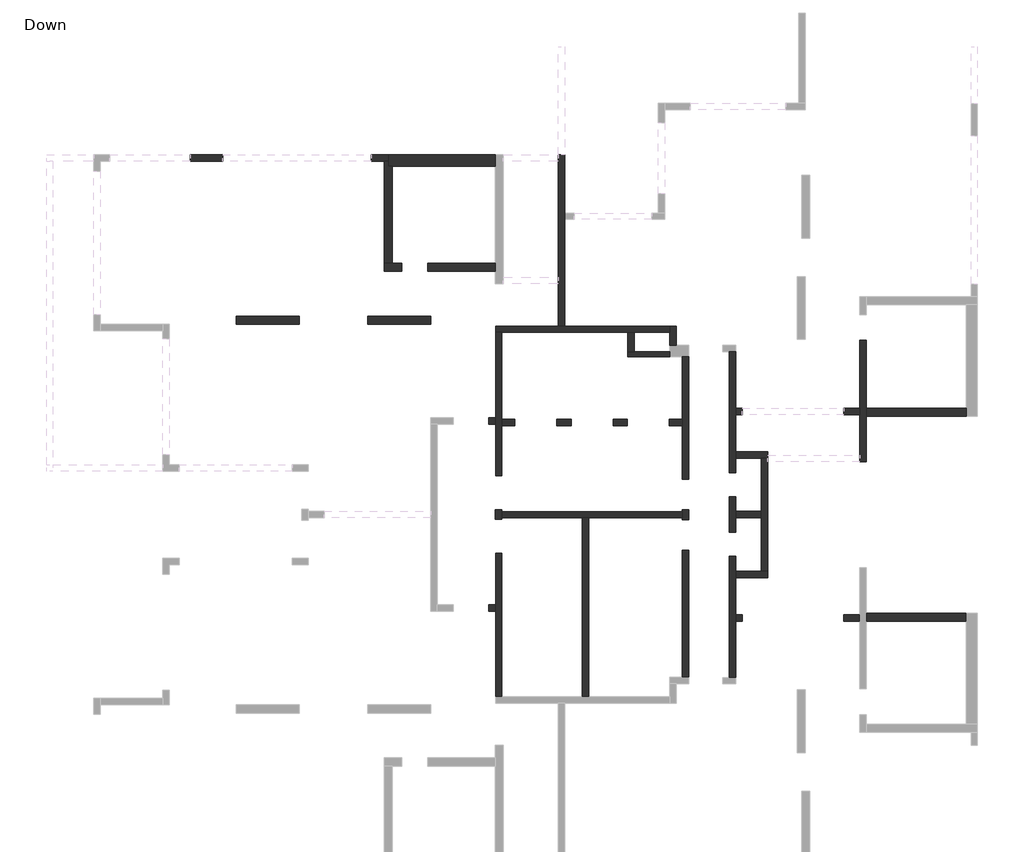
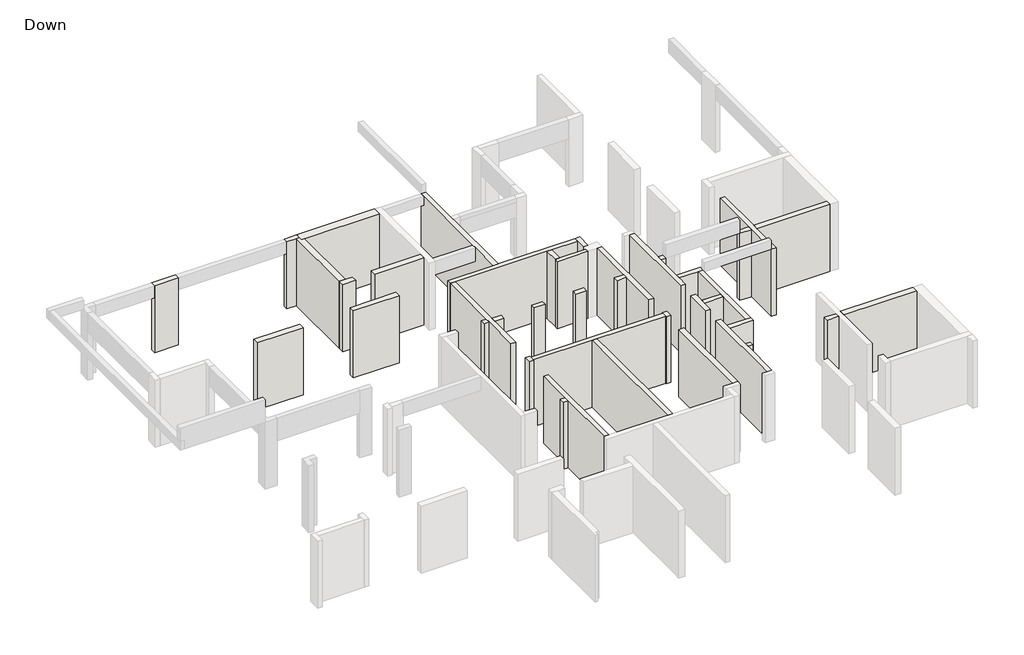
# One storey, part 2 of 3: 42 walls.
"""IFC4 building model written with IfcOpenShell, lengths in millimetres."""

from ifc_helpers import new_model, si_unit, origin, origin_with_axes, place, context, project, spatial, polyline, outline, extrude, faceted_brep, element, save

model = new_model("IFC4")

# Units and contexts
model_context = context("Model", 3, world=origin())
ifc_project = project(units=[si_unit("LENGTHUNIT", "METRE", prefix="MILLI")], contexts=[model_context])

# Site, building, storey
site = spatial("IfcSite", under=ifc_project)
building = spatial("IfcBuilding", under=site)
storey = spatial("IfcBuildingStorey", under=building, Name="Down", Elevation=0.0)

# Walls
placement = place(None, origin())
element("IfcWall", 1, ObjectType="15", at=placement, inside=storey, context=model_context, shape_type="Brep", body=[
    faceted_brep([(5701.4257984, 8540.0714033, 0.0), (4601.4257984, 8540.0714033, 0.0), (4401.4257984, 8540.0714033, 0.0), (4401.4257984, 8540.0714033, 3000.0), (4601.4257984, 8540.0714033, 3000.0), (5701.4257984, 8540.0714033, 3000.0), (5701.4257984, 8390.0714033, 0.0), (5701.4257984, 8390.0714033, 3000.0), (4401.4257984, 8390.0714033, 3000.0), (4401.4257984, 8390.0714033, 0.0)], [[[0, 1, 2, 3, 4, 5]], [[6, 7, 8, 9]], [[2, 1, 0, 6, 9]], [[5, 4, 3, 8, 7]], [[3, 2, 9, 8]], [[0, 5, 7, 6]]]),
])
element("IfcWall", 2, ObjectType="20", at=placement, inside=storey, context=model_context, shape_type="Brep", body=[
    faceted_brep([(-3022.0483227, 14641.4166181, 0.0), (-3547.0483227, 14641.4166181, 0.0), (-3547.0483227, 14641.4166181, 2450.0), (-3547.0483227, 14641.4166181, 3000.0), (-3022.0483227, 14641.4166181, 3000.0), (-3022.0483227, 14441.4166181, 0.0), (-3022.0483227, 14441.4166181, 3000.0), (-3147.0483227, 14441.4166181, 3000.0), (-3547.0483227, 14441.4166181, 3000.0), (-3547.0483227, 14441.4166181, 2450.0), (-3547.0483227, 14441.4166181, 0.0), (-3147.0483227, 14441.4166181, 0.0)], [[[0, 1, 2, 3, 4]], [[5, 6, 7, 8, 9, 10, 11]], [[1, 0, 5, 11, 10]], [[3, 2, 1, 10, 9, 8]], [[4, 3, 8, 7, 6]], [[0, 4, 6, 5]]]),
])
element("IfcWall", 3, ObjectType="20", at=placement, inside=storey, context=model_context, shape_type="Brep", body=[
    faceted_brep([(-9154.7387524, 14441.4166181, 0.0), (-8149.7387524, 14441.4166181, 0.0), (-8149.7387524, 14441.4166181, 2450.0), (-8149.7387524, 14441.4166181, 3000.0), (-9154.7387524, 14441.4166181, 3000.0), (-9154.7387524, 14441.4166181, 2450.0), (-9154.7387524, 14641.4166181, 0.0), (-9154.7387524, 14641.4166181, 2450.0), (-9154.7387524, 14641.4166181, 3000.0), (-8149.7387524, 14641.4166181, 3000.0), (-8149.7387524, 14641.4166181, 2450.0), (-8149.7387524, 14641.4166181, 0.0)], [[[0, 1, 2, 3, 4, 5]], [[6, 7, 8, 9, 10, 11]], [[1, 0, 6, 11]], [[3, 2, 1, 11, 10, 9]], [[4, 3, 9, 8]], [[0, 5, 4, 8, 7, 6]]]),
])
element("IfcWall", 4, ObjectType="20", at=placement, inside=storey, context=model_context, shape_type="Brep", body=[
    faceted_brep([(2246.4257984, 14641.4166181, 0.0), (2246.4257984, 9337.0757978, 0.0), (2246.4257984, 9337.0757978, 2820.0), (2246.4257984, 9337.0757978, 3000.0), (2246.4257984, 10641.3507002, 3000.0), (2246.4257984, 10841.3507002, 3000.0), (2246.4257984, 14441.4166181, 3000.0), (2246.4257984, 14641.4166181, 3000.0), (2246.4257984, 14641.4166181, 2750.0), (2446.4257984, 14641.4166181, 0.0), (2446.4257984, 14641.4166181, 2750.0), (2446.4257984, 14641.4166181, 3000.0), (2446.4257984, 12840.2984541, 3000.0), (2446.4257984, 12640.2984541, 3000.0), (2446.4257984, 9337.0757978, 3000.0), (2446.4257984, 9337.0757978, 2820.0), (2446.4257984, 9337.0757978, 0.0), (2446.4257984, 12640.2984541, 0.0), (2446.4257984, 12840.2984541, 0.0)], [[[0, 1, 2, 3, 4, 5, 6, 7, 8]], [[9, 10, 11, 12, 13, 14, 15, 16, 17, 18]], [[1, 0, 9, 18, 17, 16]], [[7, 6, 5, 4, 3, 14, 13, 12, 11]], [[0, 8, 7, 11, 10, 9]], [[3, 2, 1, 16, 15, 14]]]),
])
element("IfcWall", 5, ObjectType="20", at=placement, inside=storey, context=model_context, shape_type="Brep", body=[
    faceted_brep([(11596.5527515, 8889.8297041, 0.0), (11596.5527515, 6791.3653486, 0.0), (11596.5527515, 6591.3653486, 0.0), (11596.5527515, 5134.8297041, 0.0), (11596.5527515, 5134.8297041, 2820.0), (11596.5527515, 5134.8297041, 3000.0), (11596.5527515, 6591.3653486, 3000.0), (11596.5527515, 6791.3653486, 3000.0), (11596.5527515, 8889.8297041, 3000.0), (11596.5527515, 8889.8297041, 2820.0), (11796.5527515, 8889.8297041, 0.0), (11796.5527515, 8889.8297041, 2820.0), (11796.5527515, 8889.8297041, 3000.0), (11796.5527515, 6791.445915, 3000.0), (11796.5527515, 6541.445915, 3000.0), (11796.5527515, 5134.8297041, 3000.0), (11796.5527515, 5134.8297041, 0.0), (11796.5527515, 6541.445915, 0.0), (11796.5527515, 6791.445915, 0.0)], [[[0, 1, 2, 3, 4, 5, 6, 7, 8, 9]], [[10, 11, 12, 13, 14, 15, 16, 17, 18]], [[3, 2, 1, 0, 10, 18, 17, 16]], [[5, 4, 3, 16, 15]], [[8, 7, 6, 5, 15, 14, 13, 12]], [[0, 9, 8, 12, 11, 10]]]),
])
element("IfcWall", 6, ObjectType="20", at=placement, inside=storey, context=model_context, shape_type="Brep", body=[
    faceted_brep([(11103.869646, 6591.3653486, 0.0), (11596.5527515, 6591.3653486, 0.0), (11596.5527515, 6591.3653486, 2820.0), (11596.5527515, 6591.3653486, 3000.0), (11103.869646, 6591.3653486, 3000.0), (11103.869646, 6591.3653486, 2820.0), (11103.869646, 6791.3653486, 0.0), (11103.869646, 6791.3653486, 2820.0), (11103.869646, 6791.3653486, 3000.0), (11596.5527515, 6791.3653486, 3000.0), (11596.5527515, 6791.3653486, 2820.0), (11596.5527515, 6791.3653486, 0.0)], [[[0, 1, 2, 3, 4, 5]], [[6, 7, 8, 9, 10, 11]], [[1, 0, 6, 11]], [[4, 3, 9, 8]], [[0, 5, 4, 8, 7, 6]], [[3, 2, 1, 11, 10, 9]]]),
])
element("IfcWall", 7, ObjectType="20", at=placement, inside=storey, context=model_context, shape_type="Brep", body=[
    faceted_brep([(5701.4257984, 9337.0757978, 0.0), (5701.4257984, 9137.0757978, 0.0), (5701.4257984, 8740.0714033, 0.0), (5701.4257984, 8740.0714033, 3000.0), (5701.4257984, 9137.0757978, 3000.0), (5701.4257984, 9337.0757978, 3000.0), (5901.4257984, 9337.0757978, 0.0), (5901.4257984, 9337.0757978, 2820.0), (5901.4257984, 9337.0757978, 3000.0), (5901.4257984, 8740.0714033, 3000.0), (5901.4257984, 8740.0714033, 2820.0), (5901.4257984, 8740.0714033, 0.0)], [[[0, 1, 2, 3, 4, 5]], [[6, 7, 8, 9, 10, 11]], [[2, 1, 0, 6, 11]], [[5, 4, 3, 9, 8]], [[3, 2, 11, 10, 9]], [[0, 5, 8, 7, 6]]]),
])
element("IfcWall", 8, ObjectType="20", at=placement, inside=storey, context=model_context, shape_type="SweptSolid", body=[
    extrude(outline(polyline([(4601.4257984, 9137.0757978), (4601.4257984, 8540.0714033), (4401.4257984, 8540.0714033), (4401.4257984, 9137.0757978), (4601.4257984, 9137.0757978)])), origin_with_axes(), (0.0, 0.0, 1.0), 3000.0),
])
element("IfcWall", 9, ObjectType="20", at=placement, inside=storey, context=model_context, shape_type="Brep", body=[
    faceted_brep([(5701.4257984, 9337.0757978, 0.0), (2446.4257984, 9337.0757978, 0.0), (2246.4257984, 9337.0757978, 0.0), (306.4257984, 9337.0757978, 0.0), (306.4257984, 9337.0757978, 2820.0), (306.4257984, 9337.0757978, 3000.0), (2246.4257984, 9337.0757978, 3000.0), (2446.4257984, 9337.0757978, 3000.0), (5701.4257984, 9337.0757978, 3000.0), (5701.4257984, 9137.0757978, 0.0), (5701.4257984, 9137.0757978, 3000.0), (4601.4257984, 9137.0757978, 3000.0), (4401.4257984, 9137.0757978, 3000.0), (506.4257984, 9137.0757978, 3000.0), (306.4257984, 9137.0757978, 3000.0), (306.4257984, 9137.0757978, 0.0), (506.4257984, 9137.0757978, 0.0), (4401.4257984, 9137.0757978, 0.0), (4601.4257984, 9137.0757978, 0.0)], [[[0, 1, 2, 3, 4, 5, 6, 7, 8]], [[9, 10, 11, 12, 13, 14, 15, 16, 17, 18]], [[3, 2, 1, 0, 9, 18, 17, 16, 15]], [[8, 7, 6, 5, 14, 13, 12, 11, 10]], [[5, 4, 3, 15, 14]], [[0, 8, 10, 9]]]),
])
element("IfcWall", 10, ObjectType="20", at=placement, inside=storey, context=model_context, shape_type="Brep", body=[
    faceted_brep([(306.4257984, 9137.0757978, 0.0), (306.4257984, 6491.5264814, 0.0), (306.4257984, 6291.5264814, 0.0), (306.4257984, 4687.0757978, 0.0), (306.4257984, 4687.0757978, 2820.0), (306.4257984, 4687.0757978, 3000.0), (306.4257984, 6291.5264814, 3000.0), (306.4257984, 6491.5264814, 3000.0), (306.4257984, 9137.0757978, 3000.0), (506.4257984, 9137.0757978, 0.0), (506.4257984, 9137.0757978, 3000.0), (506.4257984, 6439.7589033, 3000.0), (506.4257984, 6239.7589033, 3000.0), (506.4257984, 4687.0757978, 3000.0), (506.4257984, 4687.0757978, 2820.0), (506.4257984, 4687.0757978, 0.0), (506.4257984, 6239.7589033, 0.0), (506.4257984, 6439.7589033, 0.0)], [[[0, 1, 2, 3, 4, 5, 6, 7, 8]], [[9, 10, 11, 12, 13, 14, 15, 16, 17]], [[3, 2, 1, 0, 9, 17, 16, 15]], [[5, 4, 3, 15, 14, 13]], [[8, 7, 6, 5, 13, 12, 11, 10]], [[0, 8, 10, 9]]]),
])
element("IfcWall", 11, ObjectType="20", at=placement, inside=storey, context=model_context, shape_type="Brep", body=[
    faceted_brep([(506.4257984, 6239.7589033, 0.0), (900.756853, 6239.7589033, 0.0), (900.756853, 6239.7589033, 2820.0), (900.756853, 6239.7589033, 3000.0), (506.4257984, 6239.7589033, 3000.0), (506.4257984, 6239.7589033, 2820.0), (506.4257984, 6439.7589033, 0.0), (506.4257984, 6439.7589033, 3000.0), (900.756853, 6439.7589033, 3000.0), (900.756853, 6439.7589033, 2820.0), (900.756853, 6439.7589033, 0.0)], [[[0, 1, 2, 3, 4, 5]], [[6, 7, 8, 9, 10]], [[1, 0, 6, 10]], [[3, 2, 1, 10, 9, 8]], [[4, 3, 8, 7]], [[0, 5, 4, 7, 6]]]),
])
element("IfcWall", 12, ObjectType="20", at=placement, inside=storey, context=model_context, shape_type="Brep", body=[
    faceted_brep([(306.4257984, 6491.5264814, 0.0), (96.4257984, 6491.5264814, 0.0), (96.4257984, 6491.5264814, 2820.0), (96.4257984, 6491.5264814, 3000.0), (306.4257984, 6491.5264814, 3000.0), (306.4257984, 6491.5264814, 2820.0), (306.4257984, 6291.5264814, 0.0), (306.4257984, 6291.5264814, 2820.0), (306.4257984, 6291.5264814, 3000.0), (96.4257984, 6291.5264814, 3000.0), (96.4257984, 6291.5264814, 2820.0), (96.4257984, 6291.5264814, 0.0)], [[[0, 1, 2, 3, 4, 5]], [[6, 7, 8, 9, 10, 11]], [[1, 0, 6, 11]], [[3, 2, 1, 11, 10, 9]], [[4, 3, 9, 8]], [[0, 5, 4, 8, 7, 6]]]),
])
element("IfcWall", 13, ObjectType="20", at=placement, inside=storey, context=model_context, shape_type="Brep", body=[
    faceted_brep([(2196.5063648, 6239.7589033, 0.0), (2645.7812671, 6239.7589033, 0.0), (2645.7812671, 6239.7589033, 2820.0), (2645.7812671, 6239.7589033, 3000.0), (2196.5063648, 6239.7589033, 3000.0), (2196.5063648, 6239.7589033, 2820.0), (2196.5063648, 6439.7589033, 0.0), (2196.5063648, 6439.7589033, 2820.0), (2196.5063648, 6439.7589033, 3000.0), (2645.7812671, 6439.7589033, 3000.0), (2645.7812671, 6439.7589033, 2820.0), (2645.7812671, 6439.7589033, 0.0)], [[[0, 1, 2, 3, 4, 5]], [[6, 7, 8, 9, 10, 11]], [[1, 0, 6, 11]], [[3, 2, 1, 11, 10, 9]], [[4, 3, 9, 8]], [[0, 5, 4, 8, 7, 6]]]),
])
element("IfcWall", 14, ObjectType="20", at=placement, inside=storey, context=model_context, shape_type="Brep", body=[
    faceted_brep([(3950.197771, 6239.7589033, 0.0), (4397.3022632, 6239.7589033, 0.0), (4397.3022632, 6239.7589033, 2820.0), (4397.3022632, 6239.7589033, 3000.0), (3950.197771, 6239.7589033, 3000.0), (3950.197771, 6239.7589033, 2820.0), (3950.197771, 6439.7589033, 0.0), (3950.197771, 6439.7589033, 2820.0), (3950.197771, 6439.7589033, 3000.0), (4397.3022632, 6439.7589033, 3000.0), (4397.3022632, 6439.7589033, 2820.0), (4397.3022632, 6439.7589033, 0.0)], [[[0, 1, 2, 3, 4, 5]], [[6, 7, 8, 9, 10, 11]], [[1, 0, 6, 11]], [[3, 2, 1, 11, 10, 9]], [[4, 3, 9, 8]], [[0, 5, 4, 8, 7, 6]]]),
])
element("IfcWall", 15, ObjectType="20", at=placement, inside=storey, context=model_context, shape_type="Brep", body=[
    faceted_brep([(5697.3779468, 6239.7589033, 0.0), (6096.4111499, 6239.7589033, 0.0), (6096.4111499, 6239.7589033, 2820.0), (6096.4111499, 6239.7589033, 3000.0), (5697.3779468, 6239.7589033, 3000.0), (5697.3779468, 6239.7589033, 2820.0), (5697.3779468, 6439.7589033, 0.0), (5697.3779468, 6439.7589033, 2820.0), (5697.3779468, 6439.7589033, 3000.0), (6096.4111499, 6439.7589033, 3000.0), (6096.4111499, 6439.7589033, 0.0)], [[[0, 1, 2, 3, 4, 5]], [[6, 7, 8, 9, 10]], [[1, 0, 6, 10]], [[4, 3, 9, 8]], [[0, 5, 4, 8, 7, 6]], [[3, 2, 1, 10, 9]]]),
])
element("IfcWall", 16, ObjectType="20", at=placement, inside=storey, context=model_context, shape_type="Brep", body=[
    faceted_brep([(6296.4111499, 4590.2471845, 0.0), (6296.4111499, 8390.0714033, 0.0), (6296.4111499, 8390.0714033, 3000.0), (6296.4111499, 4590.2471845, 3000.0), (6296.4111499, 4590.2471845, 2820.0), (6096.4111499, 4590.2471845, 0.0), (6096.4111499, 4590.2471845, 2820.0), (6096.4111499, 4590.2471845, 3000.0), (6096.4111499, 6239.7589033, 3000.0), (6096.4111499, 6439.7589033, 3000.0), (6096.4111499, 8390.0714033, 3000.0), (6096.4111499, 8390.0714033, 0.0), (6096.4111499, 6439.7589033, 0.0), (6096.4111499, 6239.7589033, 0.0)], [[[0, 1, 2, 3, 4]], [[5, 6, 7, 8, 9, 10, 11, 12, 13]], [[1, 0, 5, 13, 12, 11]], [[3, 2, 10, 9, 8, 7]], [[0, 4, 3, 7, 6, 5]], [[2, 1, 11, 10]]]),
])
element("IfcWall", 17, ObjectType="20", at=placement, inside=storey, context=model_context, shape_type="Brep", body=[
    faceted_brep([(7551.2304859, 8540.3936689, 0.0), (7551.2304859, 4780.3936689, 0.0), (7551.2304859, 4780.3936689, 2820.0), (7551.2304859, 4780.3936689, 3000.0), (7551.2304859, 8540.3936689, 3000.0), (7551.2304859, 8540.3936689, 2820.0), (7751.2304859, 8540.3936689, 0.0), (7751.2304859, 8540.3936689, 3000.0), (7751.2304859, 6791.3653486, 3000.0), (7751.2304859, 6591.3653486, 3000.0), (7751.2304859, 5441.3702314, 3000.0), (7751.2304859, 5241.3702314, 3000.0), (7751.2304859, 4780.3936689, 3000.0), (7751.2304859, 4780.3936689, 2820.0), (7751.2304859, 4780.3936689, 0.0), (7751.2304859, 5241.3702314, 0.0), (7751.2304859, 5441.3702314, 0.0), (7751.2304859, 6591.3653486, 0.0), (7751.2304859, 6791.3653486, 0.0)], [[[0, 1, 2, 3, 4, 5]], [[6, 7, 8, 9, 10, 11, 12, 13, 14, 15, 16, 17, 18]], [[1, 0, 6, 18, 17, 16, 15, 14]], [[3, 2, 1, 14, 13, 12]], [[4, 3, 12, 11, 10, 9, 8, 7]], [[0, 5, 4, 7, 6]]]),
])
element("IfcWall", 18, ObjectType="20", at=placement, inside=storey, context=model_context, shape_type="Brep", body=[
    faceted_brep([(7751.2304859, 5241.3702314, 0.0), (8550.5859546, 5241.3702314, 0.0), (8750.5859546, 5241.3702314, 0.0), (8750.5859546, 5241.3702314, 3000.0), (8550.5859546, 5241.3702314, 3000.0), (7751.2304859, 5241.3702314, 3000.0), (7751.2304859, 5241.3702314, 2820.0), (7751.2304859, 5441.3702314, 0.0), (7751.2304859, 5441.3702314, 2820.0), (7751.2304859, 5441.3702314, 3000.0), (8750.5859546, 5441.3702314, 3000.0), (8750.5859546, 5441.3702314, 2820.0), (8750.5859546, 5441.3702314, 0.0)], [[[0, 1, 2, 3, 4, 5, 6]], [[7, 8, 9, 10, 11, 12]], [[2, 1, 0, 7, 12]], [[5, 4, 3, 10, 9]], [[0, 6, 5, 9, 8, 7]], [[3, 2, 12, 11, 10]]]),
])
element("IfcWall", 19, ObjectType="20", at=placement, inside=storey, context=model_context, shape_type="Brep", body=[
    faceted_brep([(8550.5859546, 5241.3702314, 0.0), (8550.5859546, 3593.6505048, 0.0), (8550.5859546, 3586.3702314, 0.0), (8550.5859546, 3386.3702314, 0.0), (8550.5859546, 1738.6505048, 0.0), (8550.5859546, 1738.6505048, 2820.0), (8550.5859546, 1738.6505048, 3000.0), (8550.5859546, 3386.3702314, 3000.0), (8550.5859546, 3586.3702314, 3000.0), (8550.5859546, 3593.6505048, 3000.0), (8550.5859546, 5241.3702314, 3000.0), (8550.5859546, 5241.3702314, 2820.0), (8750.5859546, 5241.3702314, 0.0), (8750.5859546, 5241.3702314, 3000.0), (8750.5859546, 5134.8297041, 3000.0), (8750.5859546, 1845.1910322, 3000.0), (8750.5859546, 1738.6505048, 3000.0), (8750.5859546, 1738.6505048, 0.0)], [[[0, 1, 2, 3, 4, 5, 6, 7, 8, 9, 10, 11]], [[12, 13, 14, 15, 16, 17]], [[4, 3, 2, 1, 0, 12, 17]], [[10, 9, 8, 7, 6, 16, 15, 14, 13]], [[0, 11, 10, 13, 12]], [[6, 5, 4, 17, 16]]]),
])
element("IfcWall", 20, ObjectType="20", at=placement, inside=storey, context=model_context, shape_type="Brep", body=[
    faceted_brep([(8550.5859546, 3586.3702314, 0.0), (7750.5859546, 3586.3702314, 0.0), (7750.5859546, 3586.3702314, 3000.0), (8550.5859546, 3586.3702314, 3000.0), (8550.5859546, 3386.3702314, 0.0), (8550.5859546, 3386.3702314, 2820.0), (8550.5859546, 3386.3702314, 3000.0), (7750.5859546, 3386.3702314, 3000.0), (7750.5859546, 3386.3702314, 2820.0), (7750.5859546, 3386.3702314, 0.0)], [[[0, 1, 2, 3]], [[4, 5, 6, 7, 8, 9]], [[1, 0, 4, 9]], [[3, 2, 7, 6]], [[0, 3, 6, 5, 4]], [[2, 1, 9, 8, 7]]]),
])
element("IfcWall", 21, ObjectType="20", at=placement, inside=storey, context=model_context, shape_type="Brep", body=[
    faceted_brep([(7750.5859546, 2943.6505048, 0.0), (7750.5859546, 3386.3702314, 0.0), (7750.5859546, 3586.3702314, 0.0), (7750.5859546, 3593.6505048, 0.0), (7750.5859546, 4036.3702314, 0.0), (7750.5859546, 4036.3702314, 2820.0), (7750.5859546, 4036.3702314, 3000.0), (7750.5859546, 3593.6505048, 3000.0), (7750.5859546, 3586.3702314, 3000.0), (7750.5859546, 3386.3702314, 3000.0), (7750.5859546, 2943.6505048, 3000.0), (7750.5859546, 2943.6505048, 2820.0), (7550.5859546, 2943.6505048, 0.0), (7550.5859546, 2943.6505048, 2820.0), (7550.5859546, 2943.6505048, 3000.0), (7550.5859546, 4036.3702314, 3000.0), (7550.5859546, 4036.3702314, 2820.0), (7550.5859546, 4036.3702314, 0.0)], [[[0, 1, 2, 3, 4, 5, 6, 7, 8, 9, 10, 11]], [[12, 13, 14, 15, 16, 17]], [[4, 3, 2, 1, 0, 12, 17]], [[6, 5, 4, 17, 16, 15]], [[10, 9, 8, 7, 6, 15, 14]], [[0, 11, 10, 14, 13, 12]]]),
])
element("IfcWall", 22, ObjectType="20", at=placement, inside=storey, context=model_context, shape_type="Brep", body=[
    faceted_brep([(7751.2304859, 6591.3653486, 0.0), (7955.5859546, 6591.3653486, 0.0), (7955.5859546, 6591.3653486, 2820.0), (7955.5859546, 6591.3653486, 3000.0), (7751.2304859, 6591.3653486, 3000.0), (7751.2304859, 6591.3653486, 2820.0), (7751.2304859, 6791.3653486, 0.0), (7751.2304859, 6791.3653486, 2820.0), (7751.2304859, 6791.3653486, 3000.0), (7955.5859546, 6791.3653486, 3000.0), (7955.5859546, 6791.3653486, 2820.0), (7955.5859546, 6791.3653486, 0.0)], [[[0, 1, 2, 3, 4, 5]], [[6, 7, 8, 9, 10, 11]], [[1, 0, 6, 11]], [[3, 2, 1, 11, 10, 9]], [[4, 3, 9, 8]], [[0, 5, 4, 8, 7, 6]]]),
])
element("IfcWall", 23, ObjectType="20", at=placement, inside=storey, context=model_context, shape_type="Brep", body=[
    faceted_brep([(11103.869646, 188.6553877, 0.0), (11596.5527515, 188.6553877, 0.0), (11596.5527515, 188.6553877, 2820.0), (11596.5527515, 188.6553877, 3000.0), (11103.869646, 188.6553877, 3000.0), (11103.869646, 188.6553877, 2820.0), (11103.869646, 388.6553877, 0.0), (11103.869646, 388.6553877, 2820.0), (11103.869646, 388.6553877, 3000.0), (11596.5527515, 388.6553877, 3000.0), (11596.5527515, 388.6553877, 0.0)], [[[0, 1, 2, 3, 4, 5]], [[6, 7, 8, 9, 10]], [[1, 0, 6, 10]], [[4, 3, 9, 8]], [[0, 5, 4, 8, 7, 6]], [[3, 2, 1, 10, 9]]]),
])
element("IfcWall", 24, ObjectType="20", at=placement, inside=storey, context=model_context, shape_type="Brep", body=[
    faceted_brep([(506.4257984, -2157.0550616, 0.0), (506.4257984, 2292.9449384, 0.0), (506.4257984, 2292.9449384, 3000.0), (506.4257984, -2157.0550616, 3000.0), (306.4257984, -2157.0550616, 0.0), (306.4257984, -2157.0550616, 3000.0), (306.4257984, 488.4942548, 3000.0), (306.4257984, 688.4942548, 3000.0), (306.4257984, 2292.9449384, 3000.0), (306.4257984, 2292.9449384, 2820.0), (306.4257984, 2292.9449384, 0.0), (306.4257984, 688.4942548, 0.0), (306.4257984, 488.4942548, 0.0)], [[[0, 1, 2, 3]], [[4, 5, 6, 7, 8, 9, 10, 11, 12]], [[1, 0, 4, 12, 11, 10]], [[2, 1, 10, 9, 8]], [[3, 2, 8, 7, 6, 5]], [[0, 3, 5, 4]]]),
])
element("IfcWall", 25, ObjectType="20", at=placement, inside=storey, context=model_context, shape_type="Brep", body=[
    faceted_brep([(306.4257984, 688.4942548, 0.0), (96.4257984, 688.4942548, 0.0), (96.4257984, 688.4942548, 2820.0), (96.4257984, 688.4942548, 3000.0), (306.4257984, 688.4942548, 3000.0), (306.4257984, 688.4942548, 2820.0), (306.4257984, 488.4942548, 0.0), (306.4257984, 488.4942548, 2820.0), (306.4257984, 488.4942548, 3000.0), (96.4257984, 488.4942548, 3000.0), (96.4257984, 488.4942548, 2820.0), (96.4257984, 488.4942548, 0.0)], [[[0, 1, 2, 3, 4, 5]], [[6, 7, 8, 9, 10, 11]], [[1, 0, 6, 11]], [[3, 2, 1, 11, 10, 9]], [[4, 3, 9, 8]], [[0, 5, 4, 8, 7, 6]]]),
])
element("IfcWall", 26, ObjectType="20", at=placement, inside=storey, context=model_context, shape_type="Brep", body=[
    faceted_brep([(6096.4111499, 2389.7735517, 0.0), (6096.4111499, -1559.7284014, 0.0), (6096.4111499, -1559.7284014, 3000.0), (6096.4111499, 2389.4512861, 3000.0), (6096.4111499, 2389.7735517, 3000.0), (6096.4111499, 2389.7735517, 2820.0), (6296.4111499, 2389.7735517, 0.0), (6296.4111499, 2389.7735517, 2820.0), (6296.4111499, 2389.7735517, 3000.0), (6296.4111499, -1559.7284014, 3000.0), (6296.4111499, -1559.7284014, 0.0)], [[[0, 1, 2, 3, 4, 5]], [[6, 7, 8, 9, 10]], [[1, 0, 6, 10]], [[4, 3, 2, 9, 8]], [[0, 5, 4, 8, 7, 6]], [[2, 1, 10, 9]]]),
])
element("IfcWall", 27, ObjectType="20", at=placement, inside=storey, context=model_context, shape_type="Brep", body=[
    faceted_brep([(7751.2304859, -1560.3729327, 0.0), (7751.2304859, 188.6553877, 0.0), (7751.2304859, 388.6553877, 0.0), (7751.2304859, 1538.6505048, 0.0), (7751.2304859, 1738.6505048, 0.0), (7751.2304859, 2199.6270673, 0.0), (7751.2304859, 2199.6270673, 2820.0), (7751.2304859, 2199.6270673, 3000.0), (7751.2304859, 1738.6505048, 3000.0), (7751.2304859, 1538.6505048, 3000.0), (7751.2304859, 388.6553877, 3000.0), (7751.2304859, 188.6553877, 3000.0), (7751.2304859, -1560.3729327, 3000.0), (7551.2304859, -1560.3729327, 0.0), (7551.2304859, -1560.3729327, 3000.0), (7551.2304859, 2199.6270673, 3000.0), (7551.2304859, 2199.6270673, 2820.0), (7551.2304859, 2199.6270673, 0.0)], [[[0, 1, 2, 3, 4, 5, 6, 7, 8, 9, 10, 11, 12]], [[13, 14, 15, 16, 17]], [[5, 4, 3, 2, 1, 0, 13, 17]], [[7, 6, 5, 17, 16, 15]], [[12, 11, 10, 9, 8, 7, 15, 14]], [[0, 12, 14, 13]]]),
])
element("IfcWall", 28, ObjectType="20", at=placement, inside=storey, context=model_context, shape_type="Brep", body=[
    faceted_brep([(7751.2304859, 1538.6505048, 0.0), (8750.5859546, 1538.6505048, 0.0), (8750.5859546, 1538.6505048, 2820.0), (8750.5859546, 1538.6505048, 3000.0), (7751.2304859, 1538.6505048, 3000.0), (7751.2304859, 1538.6505048, 2820.0), (7751.2304859, 1738.6505048, 0.0), (7751.2304859, 1738.6505048, 2820.0), (7751.2304859, 1738.6505048, 3000.0), (8550.5859546, 1738.6505048, 3000.0), (8750.5859546, 1738.6505048, 3000.0), (8750.5859546, 1738.6505048, 0.0), (8550.5859546, 1738.6505048, 0.0)], [[[0, 1, 2, 3, 4, 5]], [[6, 7, 8, 9, 10, 11, 12]], [[1, 0, 6, 12, 11]], [[4, 3, 10, 9, 8]], [[0, 5, 4, 8, 7, 6]], [[3, 2, 1, 11, 10]]]),
])
element("IfcWall", 29, ObjectType="20", at=placement, inside=storey, context=model_context, shape_type="Brep", body=[
    faceted_brep([(8550.5859546, 3593.6505048, 0.0), (7750.5859546, 3593.6505048, 0.0), (7750.5859546, 3593.6505048, 2820.0), (7750.5859546, 3593.6505048, 3000.0), (8550.5859546, 3593.6505048, 3000.0), (8550.5859546, 3593.6505048, 2820.0), (8550.5859546, 3586.3702314, 0.0), (7750.5859546, 3586.3702314, 0.0), (7750.5859546, 3586.3702314, 3000.0), (8550.5859546, 3586.3702314, 3000.0)], [[[0, 1, 2, 3, 4, 5]], [[1, 0, 6, 7]], [[4, 3, 8, 9]], [[0, 5, 4, 9, 6]], [[3, 2, 1, 7, 8]], [[7, 6, 9, 8]]]),
])
element("IfcWall", 30, ObjectType="20", at=placement, inside=storey, context=model_context, shape_type="Brep", body=[
    faceted_brep([(7751.2304859, 188.6553877, 0.0), (7955.5859546, 188.6553877, 0.0), (7955.5859546, 188.6553877, 2820.0), (7955.5859546, 188.6553877, 3000.0), (7751.2304859, 188.6553877, 3000.0), (7751.2304859, 188.6553877, 2820.0), (7751.2304859, 388.6553877, 0.0), (7751.2304859, 388.6553877, 2820.0), (7751.2304859, 388.6553877, 3000.0), (7955.5859546, 388.6553877, 3000.0), (7955.5859546, 388.6553877, 2820.0), (7955.5859546, 388.6553877, 0.0)], [[[0, 1, 2, 3, 4, 5]], [[6, 7, 8, 9, 10, 11]], [[1, 0, 6, 11]], [[3, 2, 1, 11, 10, 9]], [[4, 3, 9, 8]], [[0, 5, 4, 8, 7, 6]]]),
])
element("IfcWall", 31, ObjectType="20", at=placement, inside=storey, context=model_context, shape_type="Brep", body=[
    faceted_brep([(501.7382984, 3340.0909345, 0.0), (501.7382984, 3385.0909345, 0.0), (501.7382984, 3585.0909345, 0.0), (501.7382984, 3635.0909345, 0.0), (501.7382984, 3635.0909345, 2820.0), (501.7382984, 3635.0909345, 3000.0), (501.7382984, 3585.0909345, 3000.0), (501.7382984, 3385.0909345, 3000.0), (501.7382984, 3340.0909345, 3000.0), (501.7382984, 3340.0909345, 2820.0), (301.7382984, 3340.0909345, 0.0), (301.7382984, 3340.0909345, 2820.0), (301.7382984, 3340.0909345, 3000.0), (301.7382984, 3635.0909345, 3000.0), (301.7382984, 3635.0909345, 2820.0), (301.7382984, 3635.0909345, 0.0), (306.4257984, 3635.0909345, 3000.0)], [[[0, 1, 2, 3, 4, 5, 6, 7, 8, 9]], [[10, 11, 12, 13, 14, 15]], [[3, 2, 1, 0, 10, 15]], [[5, 4, 3, 15, 14, 13, 16]], [[8, 7, 6, 5, 16, 13, 12]], [[0, 9, 8, 12, 11, 10]]]),
])
element("IfcWall", 32, ObjectType="20", at=placement, inside=storey, context=model_context, shape_type="Brep", body=[
    faceted_brep([(501.7382984, 3385.0909345, 0.0), (2997.0654468, 3385.0909345, 0.0), (3197.0654468, 3385.0909345, 0.0), (6101.7382984, 3385.0909345, 0.0), (6101.7382984, 3385.0909345, 2820.0), (6101.7382984, 3385.0909345, 3000.0), (3197.0654468, 3385.0909345, 3000.0), (2997.0654468, 3385.0909345, 3000.0), (501.7382984, 3385.0909345, 3000.0), (501.7382984, 3385.0909345, 2820.0), (501.7382984, 3585.0909345, 0.0), (501.7382984, 3585.0909345, 2820.0), (501.7382984, 3585.0909345, 3000.0), (6101.7382984, 3585.0909345, 3000.0), (6101.7382984, 3585.0909345, 2820.0), (6101.7382984, 3585.0909345, 0.0)], [[[0, 1, 2, 3, 4, 5, 6, 7, 8, 9]], [[10, 11, 12, 13, 14, 15]], [[3, 2, 1, 0, 10, 15]], [[8, 7, 6, 5, 13, 12]], [[0, 9, 8, 12, 11, 10]], [[5, 4, 3, 15, 14, 13]]]),
])
element("IfcWall", 33, ObjectType="20", at=placement, inside=storey, context=model_context, shape_type="Brep", body=[
    faceted_brep([(6301.7382984, 3335.0909345, 0.0), (6301.7382984, 3635.0909345, 0.0), (6301.7382984, 3635.0909345, 2820.0), (6301.7382984, 3635.0909345, 3000.0), (6301.7382984, 3335.0909345, 3000.0), (6301.7382984, 3335.0909345, 2820.0), (6101.7382984, 3335.0909345, 0.0), (6101.7382984, 3335.0909345, 2820.0), (6101.7382984, 3335.0909345, 3000.0), (6101.7382984, 3385.0909345, 3000.0), (6101.7382984, 3585.0909345, 3000.0), (6101.7382984, 3635.0909345, 3000.0), (6101.7382984, 3635.0909345, 2820.0), (6101.7382984, 3635.0909345, 0.0), (6101.7382984, 3585.0909345, 0.0), (6101.7382984, 3385.0909345, 0.0), (6296.4111499, 3635.0909345, 3000.0)], [[[0, 1, 2, 3, 4, 5]], [[6, 7, 8, 9, 10, 11, 12, 13, 14, 15]], [[1, 0, 6, 15, 14, 13]], [[3, 2, 1, 13, 12, 11, 16]], [[4, 3, 16, 11, 10, 9, 8]], [[0, 5, 4, 8, 7, 6]]]),
])
element("IfcWall", 34, ObjectType="20", at=placement, inside=storey, context=model_context, shape_type="Brep", body=[
    faceted_brep([(2997.0654468, 3385.0909345, 0.0), (2997.0654468, -2157.0550616, 0.0), (2997.0654468, -2157.0550616, 3000.0), (2997.0654468, 2292.9449384, 3000.0), (2997.0654468, 3385.0909345, 3000.0), (2997.0654468, 3385.0909345, 2820.0), (3197.0654468, 3385.0909345, 0.0), (3197.0654468, 3385.0909345, 2820.0), (3197.0654468, 3385.0909345, 3000.0), (3197.0654468, 2389.4512861, 3000.0), (3197.0654468, -2157.0550616, 3000.0), (3197.0654468, -2157.0550616, 0.0)], [[[0, 1, 2, 3, 4, 5]], [[6, 7, 8, 9, 10, 11]], [[1, 0, 6, 11]], [[4, 3, 2, 10, 9, 8]], [[0, 5, 4, 8, 7, 6]], [[2, 1, 11, 10]]]),
])
element("IfcWall", 35, ObjectType="25", at=placement, inside=storey, context=model_context, shape_type="Brep", body=[
    faceted_brep([(-7730.9496899, 9391.1944502, 0.0), (-5784.0917798, 9391.1944502, 0.0), (-5784.0917798, 9391.1944502, 2820.0), (-5784.0917798, 9391.1944502, 3000.0), (-7730.9496899, 9391.1944502, 3000.0), (-7730.9496899, 9391.1944502, 2820.0), (-7730.9496899, 9641.1944502, 0.0), (-7730.9496899, 9641.1944502, 2820.0), (-7730.9496899, 9641.1944502, 3000.0), (-5784.0917798, 9641.1944502, 3000.0), (-5784.0917798, 9641.1944502, 2820.0), (-5784.0917798, 9641.1944502, 0.0)], [[[0, 1, 2, 3, 4, 5]], [[6, 7, 8, 9, 10, 11]], [[1, 0, 6, 11]], [[3, 2, 1, 11, 10, 9]], [[4, 3, 9, 8]], [[0, 5, 4, 8, 7, 6]]]),
])
element("IfcWall", 36, ObjectType="25", at=placement, inside=storey, context=model_context, shape_type="Brep", body=[
    faceted_brep([(-3648.408186, 9391.1944502, 0.0), (-1703.720686, 9391.1944502, 0.0), (-1703.720686, 9391.1944502, 2820.0), (-1703.720686, 9391.1944502, 3000.0), (-3648.408186, 9391.1944502, 3000.0), (-3648.408186, 9391.1944502, 2820.0), (-3648.408186, 9641.1944502, 0.0), (-3648.408186, 9641.1944502, 2820.0), (-3648.408186, 9641.1944502, 3000.0), (-1703.720686, 9641.1944502, 3000.0), (-1703.720686, 9641.1944502, 2820.0), (-1703.720686, 9641.1944502, 0.0)], [[[0, 1, 2, 3, 4, 5]], [[6, 7, 8, 9, 10, 11]], [[1, 0, 6, 11]], [[3, 2, 1, 11, 10, 9]], [[4, 3, 9, 8]], [[0, 5, 4, 8, 7, 6]]]),
])
element("IfcWall", 37, ObjectType="25", at=placement, inside=storey, context=model_context, shape_type="Brep", body=[
    faceted_brep([(-1797.0483227, 11035.7061689, 0.0), (292.9516773, 11035.7061689, 0.0), (292.9516773, 11035.7061689, 2820.0), (292.9516773, 11035.7061689, 3000.0), (-1797.0483227, 11035.7061689, 3000.0), (-1797.0483227, 11035.7061689, 2820.0), (-1797.0483227, 11285.7061689, 0.0), (-1797.0483227, 11285.7061689, 2820.0), (-1797.0483227, 11285.7061689, 3000.0), (292.9516773, 11285.7061689, 3000.0), (292.9516773, 11285.7061689, 2820.0), (292.9516773, 11285.7061689, 0.0)], [[[0, 1, 2, 3, 4, 5]], [[6, 7, 8, 9, 10, 11]], [[1, 0, 6, 11]], [[4, 3, 9, 8]], [[0, 5, 4, 8, 7, 6]], [[3, 2, 1, 11, 10, 9]]]),
])
element("IfcWall", 38, ObjectType="25", at=placement, inside=storey, context=model_context, shape_type="Brep", body=[
    faceted_brep([(-3147.0483227, 14441.4166181, 0.0), (-3147.0483227, 11285.7061689, 0.0), (-3147.0483227, 11285.7061689, 3000.0), (-3147.0483227, 14441.4166181, 3000.0), (-3147.0483227, 14441.4166181, 2820.0), (-2897.0483227, 14291.4166181, 0.0), (-2897.0483227, 14291.4166181, 2820.0), (-2897.0483227, 14291.4166181, 3000.0), (-2897.0483227, 11285.7061689, 3000.0), (-2897.0483227, 11285.7061689, 2820.0), (-2897.0483227, 11285.7061689, 0.0), (-3022.0483227, 14441.4166181, 0.0), (-3022.0483227, 14291.4166181, 0.0), (-3022.0483227, 14291.4166181, 3000.0), (-3022.0483227, 14441.4166181, 3000.0)], [[[0, 1, 2, 3, 4]], [[5, 6, 7, 8, 9, 10]], [[1, 0, 11, 12, 5, 10]], [[3, 2, 8, 7, 13, 14]], [[0, 4, 3, 14, 11]], [[14, 13, 12, 11]], [[13, 7, 6, 5, 12]], [[2, 1, 10, 9, 8]]]),
])
element("IfcWall", 39, ObjectType="25", at=placement, inside=storey, context=model_context, shape_type="Brep", body=[
    faceted_brep([(-3147.0483227, 11035.7061689, 0.0), (-2602.0483227, 11035.7061689, 0.0), (-2602.0483227, 11035.7061689, 2820.0), (-2602.0483227, 11035.7061689, 3000.0), (-3147.0483227, 11035.7061689, 3000.0), (-3147.0483227, 11035.7061689, 2820.0), (-3147.0483227, 11285.7061689, 0.0), (-3147.0483227, 11285.7061689, 3000.0), (-2897.0483227, 11285.7061689, 3000.0), (-2602.0483227, 11285.7061689, 3000.0), (-2602.0483227, 11285.7061689, 2820.0), (-2602.0483227, 11285.7061689, 0.0), (-2897.0483227, 11285.7061689, 0.0)], [[[0, 1, 2, 3, 4, 5]], [[6, 7, 8, 9, 10, 11, 12]], [[1, 0, 6, 12, 11]], [[3, 2, 1, 11, 10, 9]], [[4, 3, 9, 8, 7]], [[0, 5, 4, 7, 6]]]),
])
element("IfcWall", 40, ObjectType="25", at=placement, inside=storey, context=model_context, shape_type="Brep", body=[
    faceted_brep([(14897.1826343, 6791.445915, 0.0), (11796.5527515, 6791.445915, 0.0), (11796.5527515, 6791.445915, 2820.0), (11796.5527515, 6791.445915, 3000.0), (14897.1826343, 6791.445915, 3000.0), (14897.1826343, 6791.445915, 2820.0), (14897.1826343, 6541.445915, 0.0), (14897.1826343, 6541.445915, 3000.0), (11796.5527515, 6541.445915, 3000.0), (11796.5527515, 6541.445915, 0.0)], [[[0, 1, 2, 3, 4, 5]], [[6, 7, 8, 9]], [[1, 0, 6, 9]], [[4, 3, 8, 7]], [[0, 5, 4, 7, 6]], [[3, 2, 1, 9, 8]]]),
])
element("IfcWall", 41, ObjectType="25", at=placement, inside=storey, context=model_context, shape_type="Brep", body=[
    faceted_brep([(14897.1826343, 438.5748212, 0.0), (11796.5527515, 438.5748212, 0.0), (11796.5527515, 438.5748212, 3000.0), (14897.1826343, 438.5748212, 3000.0), (14897.1826343, 188.5748212, 0.0), (14897.1826343, 188.5748212, 2820.0), (14897.1826343, 188.5748212, 3000.0), (11796.5527515, 188.5748212, 3000.0), (11796.5527515, 188.5748212, 2820.0), (11796.5527515, 188.5748212, 0.0)], [[[0, 1, 2, 3]], [[4, 5, 6, 7, 8, 9]], [[1, 0, 4, 9]], [[3, 2, 7, 6]], [[0, 3, 6, 5, 4]], [[2, 1, 9, 8, 7]]]),
])
element("IfcWall", 42, ObjectType="35", at=placement, inside=storey, context=model_context, shape_type="Brep", body=[
    faceted_brep([(292.9516773, 14641.4166181, 0.0), (-3022.0483227, 14641.4166181, 0.0), (-3022.0483227, 14641.4166181, 3000.0), (292.9516773, 14641.4166181, 3000.0), (292.9516773, 14291.4166181, 0.0), (292.9516773, 14291.4166181, 2820.0), (292.9516773, 14291.4166181, 3000.0), (-2897.0483227, 14291.4166181, 3000.0), (-3022.0483227, 14291.4166181, 3000.0), (-3022.0483227, 14291.4166181, 0.0), (-2897.0483227, 14291.4166181, 0.0), (-3022.0483227, 14441.4166181, 0.0), (-3022.0483227, 14441.4166181, 3000.0)], [[[0, 1, 2, 3]], [[4, 5, 6, 7, 8, 9, 10]], [[1, 0, 4, 10, 9, 11]], [[2, 1, 11, 9, 8, 12]], [[3, 2, 12, 8, 7, 6]], [[0, 3, 6, 5, 4]]]),
])

save(model, "model.ifc")

# Revit data of these elements
# Type "15"
#   Layers, outside or top first: 15 cm "Concrete" (function 1)
# Type "20"
#   Layers, outside or top first: 20 cm "Concrete" (function 1)
# Type "25"
#   Layers, outside or top first: 25 cm "Concrete" (function 1)
# Type "35"
#   Layers, outside or top first: 35 cm "Concrete" (function 1)
# Element 1 (IfcWall, "15")
#   Comments = ""
#   Mark = "W112"
#   SOFiSTiK_EdgeZones = "W112"
#   SOFiSTiK_AMG_Comments = ""
#   Top Offset = 0 cm
#   Base Offset = 0 cm
#   wall height = 300 cm
#   SOFiSTiK_AMG_Scheduled = yes
#   SOFiSTiK_AMG_Adjusted = yes
#   Phase Created = New Construction
#   Base Constraint = Down
#   Top Constraint = Typical Floor
#   Materials on its faces: "Concrete"
# Element 2 (IfcWall, "20")
#   Comments = ""
#   Mark = "W4"
#   SOFiSTiK_EdgeZones = "W4"
#   SOFiSTiK_AMG_Comments = ""
#   Top Offset = 0 cm
#   Base Offset = 0 cm
#   wall height = 300 cm
#   SOFiSTiK_AMG_Scheduled = yes
#   SOFiSTiK_AMG_Adjusted = yes
#   Phase Created = New Construction
#   Base Constraint = Down
#   Top Constraint = Typical Floor
#   Materials on its faces: "Concrete"
# Element 3 (IfcWall, "20")
#   Comments = ""
#   Mark = "W5"
#   SOFiSTiK_EdgeZones = "W5"
#   SOFiSTiK_AMG_Comments = ""
#   Top Offset = 0 cm
#   Base Offset = 0 cm
#   wall height = 300 cm
#   SOFiSTiK_AMG_Scheduled = yes
#   SOFiSTiK_AMG_Adjusted = yes
#   Phase Created = New Construction
#   Base Constraint = Down
#   Top Constraint = Typical Floor
#   Materials on its faces: "Concrete"
# Element 4 (IfcWall, "20")
#   Comments = ""
#   Mark = "W6"
#   SOFiSTiK_EdgeZones = "W6"
#   SOFiSTiK_AMG_Comments = ""
#   Top Offset = 0 cm
#   Base Offset = 0 cm
#   wall height = 300 cm
#   SOFiSTiK_AMG_Scheduled = yes
#   SOFiSTiK_AMG_Adjusted = yes
#   Phase Created = New Construction
#   Base Constraint = Down
#   Top Constraint = Typical Floor
#   Materials on its faces: "Concrete"
# Element 5 (IfcWall, "20")
#   Comments = ""
#   Mark = "W20"
#   SOFiSTiK_EdgeZones = "W20"
#   SOFiSTiK_AMG_Comments = ""
#   Top Offset = 0 cm
#   Base Offset = 0 cm
#   wall height = 300 cm
#   SOFiSTiK_AMG_Scheduled = yes
#   SOFiSTiK_AMG_Adjusted = yes
#   Phase Created = New Construction
#   Base Constraint = Down
#   Top Constraint = Typical Floor
#   Materials on its faces: "Concrete"
# Element 6 (IfcWall, "20")
#   Comments = ""
#   Mark = "W21"
#   SOFiSTiK_EdgeZones = "W21"
#   SOFiSTiK_AMG_Comments = ""
#   Top Offset = 0 cm
#   Base Offset = 0 cm
#   wall height = 300 cm
#   SOFiSTiK_AMG_Scheduled = yes
#   SOFiSTiK_AMG_Adjusted = yes
#   Phase Created = New Construction
#   Base Constraint = Down
#   Top Constraint = Typical Floor
#   Materials on its faces: "Concrete"
# Element 7 (IfcWall, "20")
#   Comments = ""
#   Mark = "W23"
#   SOFiSTiK_EdgeZones = "W23"
#   SOFiSTiK_AMG_Comments = ""
#   Top Offset = 0 cm
#   Base Offset = 0 cm
#   wall height = 300 cm
#   SOFiSTiK_AMG_Scheduled = yes
#   SOFiSTiK_AMG_Adjusted = yes
#   Phase Created = New Construction
#   Base Constraint = Down
#   Top Constraint = Typical Floor
#   Materials on its faces: "Concrete"
# Element 8 (IfcWall, "20")
#   Comments = ""
#   Mark = "W24"
#   SOFiSTiK_EdgeZones = "W24"
#   SOFiSTiK_AMG_Comments = ""
#   Top Offset = 0 cm
#   Base Offset = 0 cm
#   wall height = 300 cm
#   SOFiSTiK_AMG_Scheduled = yes
#   SOFiSTiK_AMG_Adjusted = yes
#   Phase Created = New Construction
#   Base Constraint = Down
#   Top Constraint = Typical Floor
#   Materials on its faces: "Concrete"
# Element 9 (IfcWall, "20")
#   Comments = ""
#   Mark = "W25"
#   SOFiSTiK_EdgeZones = "W25"
#   SOFiSTiK_AMG_Comments = ""
#   Top Offset = 0 cm
#   Base Offset = 0 cm
#   wall height = 300 cm
#   SOFiSTiK_AMG_Scheduled = yes
#   SOFiSTiK_AMG_Adjusted = yes
#   Phase Created = New Construction
#   Base Constraint = Down
#   Top Constraint = Typical Floor
#   Materials on its faces: "Concrete"
# Element 10 (IfcWall, "20")
#   Comments = ""
#   Mark = "W26"
#   SOFiSTiK_EdgeZones = "W26"
#   SOFiSTiK_AMG_Comments = ""
#   Top Offset = 0 cm
#   Base Offset = 0 cm
#   wall height = 300 cm
#   SOFiSTiK_AMG_Scheduled = yes
#   SOFiSTiK_AMG_Adjusted = yes
#   Phase Created = New Construction
#   Base Constraint = Down
#   Top Constraint = Typical Floor
#   Materials on its faces: "Concrete"
# Element 11 (IfcWall, "20")
#   Comments = ""
#   Mark = "W27"
#   SOFiSTiK_EdgeZones = "W27"
#   SOFiSTiK_AMG_Comments = ""
#   Top Offset = 0 cm
#   Base Offset = 0 cm
#   wall height = 300 cm
#   SOFiSTiK_AMG_Scheduled = yes
#   SOFiSTiK_AMG_Adjusted = yes
#   Phase Created = New Construction
#   Base Constraint = Down
#   Top Constraint = Typical Floor
#   Materials on its faces: "Concrete"
# Element 12 (IfcWall, "20")
#   Comments = ""
#   Mark = "W28"
#   SOFiSTiK_EdgeZones = "W28"
#   SOFiSTiK_AMG_Comments = ""
#   Top Offset = 0 cm
#   Base Offset = 0 cm
#   wall height = 300 cm
#   SOFiSTiK_AMG_Scheduled = yes
#   SOFiSTiK_AMG_Adjusted = yes
#   Phase Created = New Construction
#   Base Constraint = Down
#   Top Constraint = Typical Floor
#   Materials on its faces: "Concrete"
# Element 13 (IfcWall, "20")
#   Comments = ""
#   Mark = "W29"
#   SOFiSTiK_EdgeZones = "W29"
#   SOFiSTiK_AMG_Comments = ""
#   Top Offset = 0 cm
#   Base Offset = 0 cm
#   wall height = 300 cm
#   SOFiSTiK_AMG_Scheduled = yes
#   SOFiSTiK_AMG_Adjusted = yes
#   Phase Created = New Construction
#   Base Constraint = Down
#   Top Constraint = Typical Floor
#   Materials on its faces: "Concrete"
# Element 14 (IfcWall, "20")
#   Comments = ""
#   Mark = "W30"
#   SOFiSTiK_EdgeZones = "W30"
#   SOFiSTiK_AMG_Comments = ""
#   Top Offset = 0 cm
#   Base Offset = 0 cm
#   wall height = 300 cm
#   SOFiSTiK_AMG_Scheduled = yes
#   SOFiSTiK_AMG_Adjusted = yes
#   Phase Created = New Construction
#   Base Constraint = Down
#   Top Constraint = Typical Floor
#   Materials on its faces: "Concrete"
# Element 15 (IfcWall, "20")
#   Comments = ""
#   Mark = "W31"
#   SOFiSTiK_EdgeZones = "W31"
#   SOFiSTiK_AMG_Comments = ""
#   Top Offset = 0 cm
#   Base Offset = 0 cm
#   wall height = 300 cm
#   SOFiSTiK_AMG_Scheduled = yes
#   SOFiSTiK_AMG_Adjusted = yes
#   Phase Created = New Construction
#   Base Constraint = Down
#   Top Constraint = Typical Floor
#   Materials on its faces: "Concrete"
# Element 16 (IfcWall, "20")
#   Comments = ""
#   Mark = "W32"
#   SOFiSTiK_EdgeZones = "W32"
#   SOFiSTiK_AMG_Comments = ""
#   Top Offset = 0 cm
#   Base Offset = 0 cm
#   wall height = 300 cm
#   SOFiSTiK_AMG_Scheduled = yes
#   SOFiSTiK_AMG_Adjusted = yes
#   Phase Created = New Construction
#   Base Constraint = Down
#   Top Constraint = Typical Floor
#   Materials on its faces: "Concrete"
# Element 17 (IfcWall, "20")
#   Comments = ""
#   Mark = "W34"
#   SOFiSTiK_EdgeZones = "W34"
#   SOFiSTiK_AMG_Comments = ""
#   Top Offset = 0 cm
#   Base Offset = 0 cm
#   wall height = 300 cm
#   SOFiSTiK_AMG_Scheduled = yes
#   SOFiSTiK_AMG_Adjusted = yes
#   Phase Created = New Construction
#   Base Constraint = Down
#   Top Constraint = Typical Floor
#   Materials on its faces: "Concrete"
# Element 18 (IfcWall, "20")
#   Comments = ""
#   Mark = "W35"
#   SOFiSTiK_EdgeZones = "W35"
#   SOFiSTiK_AMG_Comments = ""
#   Top Offset = 0 cm
#   Base Offset = 0 cm
#   wall height = 300 cm
#   SOFiSTiK_AMG_Scheduled = yes
#   SOFiSTiK_AMG_Adjusted = yes
#   Phase Created = New Construction
#   Base Constraint = Down
#   Top Constraint = Typical Floor
#   Materials on its faces: "Concrete"
# Element 19 (IfcWall, "20")
#   Comments = ""
#   Mark = "W36"
#   SOFiSTiK_EdgeZones = "W36"
#   SOFiSTiK_AMG_Comments = ""
#   Top Offset = 0 cm
#   Base Offset = 0 cm
#   wall height = 300 cm
#   SOFiSTiK_AMG_Scheduled = yes
#   SOFiSTiK_AMG_Adjusted = yes
#   Phase Created = New Construction
#   Base Constraint = Down
#   Top Constraint = Typical Floor
#   Materials on its faces: "Concrete"
# Element 20 (IfcWall, "20")
#   Comments = ""
#   Mark = "W37"
#   SOFiSTiK_EdgeZones = "W37"
#   SOFiSTiK_AMG_Comments = ""
#   Top Offset = 0 cm
#   Base Offset = 0 cm
#   wall height = 300 cm
#   SOFiSTiK_AMG_Scheduled = yes
#   SOFiSTiK_AMG_Adjusted = yes
#   Phase Created = New Construction
#   Base Constraint = Down
#   Top Constraint = Typical Floor
#   Materials on its faces: "Concrete"
# Element 21 (IfcWall, "20")
#   Comments = ""
#   Mark = "W38"
#   SOFiSTiK_EdgeZones = "W38"
#   SOFiSTiK_AMG_Comments = ""
#   Top Offset = 0 cm
#   Base Offset = 0 cm
#   wall height = 300 cm
#   SOFiSTiK_AMG_Scheduled = yes
#   SOFiSTiK_AMG_Adjusted = yes
#   Phase Created = New Construction
#   Base Constraint = Down
#   Top Constraint = Typical Floor
#   Materials on its faces: "Concrete"
# Element 22 (IfcWall, "20")
#   Comments = ""
#   Mark = "W44"
#   SOFiSTiK_EdgeZones = "W44"
#   SOFiSTiK_AMG_Comments = ""
#   Top Offset = 0 cm
#   Base Offset = 0 cm
#   wall height = 300 cm
#   SOFiSTiK_AMG_Scheduled = yes
#   SOFiSTiK_AMG_Adjusted = yes
#   Phase Created = New Construction
#   Base Constraint = Down
#   Top Constraint = Typical Floor
#   Materials on its faces: "Concrete"
# Element 23 (IfcWall, "20")
#   Comments = ""
#   Mark = "W65"
#   SOFiSTiK_EdgeZones = "W65"
#   SOFiSTiK_AMG_Comments = ""
#   Top Offset = 0 cm
#   Base Offset = 0 cm
#   wall height = 300 cm
#   SOFiSTiK_AMG_Scheduled = yes
#   SOFiSTiK_AMG_Adjusted = yes
#   Phase Created = New Construction
#   Base Constraint = Down
#   Top Constraint = Typical Floor
#   Materials on its faces: "Concrete"
# Element 24 (IfcWall, "20")
#   Comments = ""
#   Mark = "W69"
#   SOFiSTiK_EdgeZones = "W69"
#   SOFiSTiK_AMG_Comments = ""
#   Top Offset = 0 cm
#   Base Offset = 0 cm
#   wall height = 300 cm
#   SOFiSTiK_AMG_Scheduled = yes
#   SOFiSTiK_AMG_Adjusted = yes
#   Phase Created = New Construction
#   Base Constraint = Down
#   Top Constraint = Typical Floor
#   Materials on its faces: "Concrete"
# Element 25 (IfcWall, "20")
#   Comments = ""
#   Mark = "W70"
#   SOFiSTiK_EdgeZones = "W70"
#   SOFiSTiK_AMG_Comments = ""
#   Top Offset = 0 cm
#   Base Offset = 0 cm
#   wall height = 300 cm
#   SOFiSTiK_AMG_Scheduled = yes
#   SOFiSTiK_AMG_Adjusted = yes
#   Phase Created = New Construction
#   Base Constraint = Down
#   Top Constraint = Typical Floor
#   Materials on its faces: "Concrete"
# Element 26 (IfcWall, "20")
#   Comments = ""
#   Mark = "W71"
#   SOFiSTiK_EdgeZones = "W71"
#   SOFiSTiK_AMG_Comments = ""
#   Top Offset = 0 cm
#   Base Offset = 0 cm
#   wall height = 300 cm
#   SOFiSTiK_AMG_Scheduled = yes
#   SOFiSTiK_AMG_Adjusted = yes
#   Phase Created = New Construction
#   Base Constraint = Down
#   Top Constraint = Typical Floor
#   Materials on its faces: "Concrete"
# Element 27 (IfcWall, "20")
#   Comments = ""
#   Mark = "W73"
#   SOFiSTiK_EdgeZones = "W73"
#   SOFiSTiK_AMG_Comments = ""
#   Top Offset = 0 cm
#   Base Offset = 0 cm
#   wall height = 300 cm
#   SOFiSTiK_AMG_Scheduled = yes
#   SOFiSTiK_AMG_Adjusted = yes
#   Phase Created = New Construction
#   Base Constraint = Down
#   Top Constraint = Typical Floor
#   Materials on its faces: "Concrete"
# Element 28 (IfcWall, "20")
#   Comments = ""
#   Mark = "W74"
#   SOFiSTiK_EdgeZones = "W74"
#   SOFiSTiK_AMG_Comments = ""
#   Top Offset = 0 cm
#   Base Offset = 0 cm
#   wall height = 300 cm
#   SOFiSTiK_AMG_Scheduled = yes
#   SOFiSTiK_AMG_Adjusted = yes
#   Phase Created = New Construction
#   Base Constraint = Down
#   Top Constraint = Typical Floor
#   Materials on its faces: "Concrete"
# Element 29 (IfcWall, "20")
#   Comments = ""
#   Mark = "W76"
#   SOFiSTiK_EdgeZones = "W76"
#   SOFiSTiK_AMG_Comments = ""
#   Top Offset = 0 cm
#   Base Offset = 0 cm
#   wall height = 300 cm
#   SOFiSTiK_AMG_Scheduled = yes
#   SOFiSTiK_AMG_Adjusted = yes
#   Phase Created = New Construction
#   Base Constraint = Down
#   Top Constraint = Typical Floor
#   Materials on its faces: "Concrete"
# Element 30 (IfcWall, "20")
#   Comments = ""
#   Mark = "W78"
#   SOFiSTiK_EdgeZones = "W78"
#   SOFiSTiK_AMG_Comments = ""
#   Top Offset = 0 cm
#   Base Offset = 0 cm
#   wall height = 300 cm
#   SOFiSTiK_AMG_Scheduled = yes
#   SOFiSTiK_AMG_Adjusted = yes
#   Phase Created = New Construction
#   Base Constraint = Down
#   Top Constraint = Typical Floor
#   Materials on its faces: "Concrete"
# Element 31 (IfcWall, "20")
#   Comments = ""
#   Mark = "W80"
#   SOFiSTiK_EdgeZones = "W80"
#   SOFiSTiK_AMG_Comments = ""
#   Top Offset = 0 cm
#   Base Offset = 0 cm
#   wall height = 300 cm
#   SOFiSTiK_AMG_Scheduled = yes
#   SOFiSTiK_AMG_Adjusted = yes
#   Phase Created = New Construction
#   Base Constraint = Down
#   Top Constraint = Typical Floor
#   Materials on its faces: "Concrete"
# Element 32 (IfcWall, "20")
#   Comments = ""
#   Mark = "W81"
#   SOFiSTiK_EdgeZones = "W81"
#   SOFiSTiK_AMG_Comments = ""
#   Top Offset = 0 cm
#   Base Offset = 0 cm
#   wall height = 300 cm
#   SOFiSTiK_AMG_Scheduled = yes
#   SOFiSTiK_AMG_Adjusted = yes
#   Phase Created = New Construction
#   Base Constraint = Down
#   Top Constraint = Typical Floor
#   Materials on its faces: "Concrete"
# Element 33 (IfcWall, "20")
#   Comments = ""
#   Mark = "W82"
#   SOFiSTiK_EdgeZones = "W82"
#   SOFiSTiK_AMG_Comments = ""
#   Top Offset = 0 cm
#   Base Offset = 0 cm
#   wall height = 300 cm
#   SOFiSTiK_AMG_Scheduled = yes
#   SOFiSTiK_AMG_Adjusted = yes
#   Phase Created = New Construction
#   Base Constraint = Down
#   Top Constraint = Typical Floor
#   Materials on its faces: "Concrete"
# Element 34 (IfcWall, "20")
#   Comments = ""
#   Mark = "W84"
#   SOFiSTiK_EdgeZones = "W84"
#   SOFiSTiK_AMG_Comments = ""
#   Top Offset = 0 cm
#   Base Offset = 0 cm
#   wall height = 300 cm
#   SOFiSTiK_AMG_Scheduled = yes
#   SOFiSTiK_AMG_Adjusted = yes
#   Phase Created = New Construction
#   Base Constraint = Down
#   Top Constraint = Typical Floor
#   Materials on its faces: "Concrete"
# Element 35 (IfcWall, "25")
#   Comments = ""
#   Mark = "W85"
#   SOFiSTiK_EdgeZones = "W85"
#   SOFiSTiK_AMG_Comments = ""
#   Top Offset = 0 cm
#   Base Offset = 0 cm
#   wall height = 300 cm
#   SOFiSTiK_AMG_Scheduled = yes
#   SOFiSTiK_AMG_Adjusted = yes
#   Phase Created = New Construction
#   Base Constraint = Down
#   Top Constraint = Typical Floor
#   Materials on its faces: "Concrete"
# Element 36 (IfcWall, "25")
#   Comments = ""
#   Mark = "W86"
#   SOFiSTiK_EdgeZones = "W86"
#   SOFiSTiK_AMG_Comments = ""
#   Top Offset = 0 cm
#   Base Offset = 0 cm
#   wall height = 300 cm
#   SOFiSTiK_AMG_Scheduled = yes
#   SOFiSTiK_AMG_Adjusted = yes
#   Phase Created = New Construction
#   Base Constraint = Down
#   Top Constraint = Typical Floor
#   Materials on its faces: "Concrete"
# Element 37 (IfcWall, "25")
#   Comments = ""
#   Mark = "W87"
#   SOFiSTiK_EdgeZones = "W87"
#   SOFiSTiK_AMG_Comments = ""
#   Top Offset = 0 cm
#   Base Offset = 0 cm
#   wall height = 300 cm
#   SOFiSTiK_AMG_Scheduled = yes
#   SOFiSTiK_AMG_Adjusted = yes
#   Phase Created = New Construction
#   Base Constraint = Down
#   Top Constraint = Typical Floor
#   Materials on its faces: "Concrete"
# Element 38 (IfcWall, "25")
#   Comments = ""
#   Mark = "W89"
#   SOFiSTiK_EdgeZones = "W89"
#   SOFiSTiK_AMG_Comments = ""
#   Top Offset = 0 cm
#   Base Offset = 0 cm
#   wall height = 300 cm
#   SOFiSTiK_AMG_Scheduled = yes
#   SOFiSTiK_AMG_Adjusted = yes
#   Phase Created = New Construction
#   Base Constraint = Down
#   Top Constraint = Typical Floor
#   Materials on its faces: "Concrete"
# Element 39 (IfcWall, "25")
#   Comments = ""
#   Mark = "W90"
#   SOFiSTiK_EdgeZones = "W90"
#   SOFiSTiK_AMG_Comments = ""
#   Top Offset = 0 cm
#   Base Offset = 0 cm
#   wall height = 300 cm
#   SOFiSTiK_AMG_Scheduled = yes
#   SOFiSTiK_AMG_Adjusted = yes
#   Phase Created = New Construction
#   Base Constraint = Down
#   Top Constraint = Typical Floor
#   Materials on its faces: "Concrete"
# Element 40 (IfcWall, "25")
#   Comments = ""
#   Mark = "W95"
#   SOFiSTiK_EdgeZones = "W95"
#   SOFiSTiK_AMG_Comments = ""
#   Top Offset = 0 cm
#   Base Offset = 0 cm
#   wall height = 300 cm
#   SOFiSTiK_AMG_Scheduled = yes
#   SOFiSTiK_AMG_Adjusted = yes
#   Phase Created = New Construction
#   Base Constraint = Down
#   Top Constraint = Typical Floor
#   Materials on its faces: "Concrete"
# Element 41 (IfcWall, "25")
#   Comments = ""
#   Mark = "W106"
#   SOFiSTiK_EdgeZones = "W106"
#   SOFiSTiK_AMG_Comments = ""
#   Top Offset = 0 cm
#   Base Offset = 0 cm
#   wall height = 300 cm
#   SOFiSTiK_AMG_Scheduled = yes
#   SOFiSTiK_AMG_Adjusted = yes
#   Phase Created = New Construction
#   Base Constraint = Down
#   Top Constraint = Typical Floor
#   Materials on its faces: "Concrete"
# Element 42 (IfcWall, "35")
#   Comments = ""
#   Mark = "W107"
#   SOFiSTiK_EdgeZones = "W107"
#   SOFiSTiK_AMG_Comments = ""
#   Top Offset = 0 cm
#   Base Offset = 0 cm
#   wall height = 300 cm
#   SOFiSTiK_AMG_Scheduled = yes
#   SOFiSTiK_AMG_Adjusted = yes
#   Phase Created = New Construction
#   Base Constraint = Down
#   Top Constraint = Typical Floor
#   Materials on its faces: "Concrete"
# Materials
#   "Concrete": class "Concrete", colour RGB 192 192 192, transparency 0, Keynote = "01000", Description = "Cast-in-place concrete", Cost = 0
